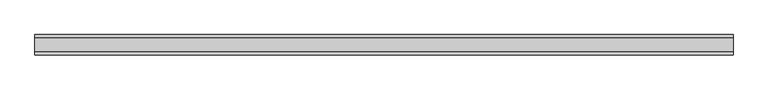
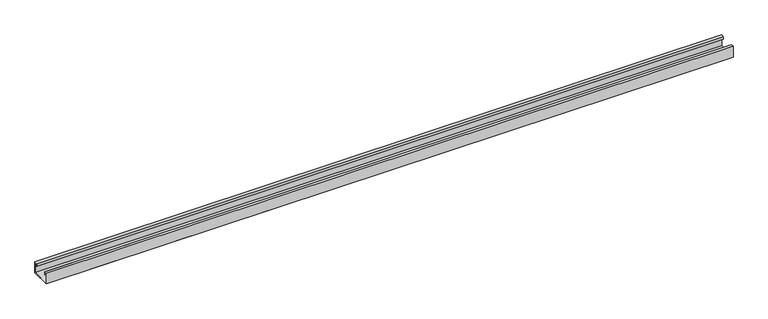
"""IFC4 building model written with IfcOpenShell, lengths in millimetres: proxy geometry, Generic Models 7:Generic Models 1:1:Generic Models 1:1 : Generic Models 7:Generic Models 1:337419:57 : Generic Models 7:Generic Models 1:1:Generic Models 1:1 : Generic Models 7:Generic Models 1:337419:306201."""

from ifc_helpers import new_model, si_unit, frame, origin, place, context, project, spatial, polyline, outline, extrude, source, transform, mapped, element, save


def generic_models_7ddd9d2e(model_context):
    return source(origin(), model_context, "Body", "SweptSolid", [
        extrude(outline(polyline([(-578792.9131695, 2440.1859375), (-579005.2695987, 2440.1859375), (-579005.2695987, 2561.318129), (-578973.5195987, 2561.318129), (-578973.5195987, 2529.568129), (-578976.4229092, 2529.568129), (-578976.4229092, 2558.4148184), (-579002.3662881, 2558.4148184), (-579002.3662881, 2443.0892481), (-578795.8164801, 2443.0892481), (-578795.8164801, 2558.4148184), (-578821.7598589, 2558.4148184), (-578821.7598589, 2529.568129), (-578824.6631695, 2529.568129), (-578824.6631695, 2561.318129), (-578792.9131695, 2561.318129), (-578792.9131695, 2440.1859375)])), frame((588867.6367239, 0.0, 0.0), z_axis=(1.0, 0.0, 0.0), x_axis=(0.0, 1.0, 0.0)), (0.0, 0.0, 1.0), 7315.2),
    ])


if __name__ == "__main__":
    model = new_model("IFC4")
    model_context = context("Model", 3, world=origin())
    ifc_project = project(units=[si_unit("LENGTHUNIT", "METRE", prefix="MILLI")], contexts=[model_context])
    site = spatial("IfcSite", under=ifc_project)
    building = spatial("IfcBuilding", under=site)
    placement = place(None, origin())
    generic_models_shape = generic_models_7ddd9d2e(model_context)
    element("IfcBuildingElementProxy", 1, Name="Generic Models 7:Generic Models 1:1:Generic Models 1:1 : Generic Models 7:Generic Models 1:337419:57 : Generic Models 7:Generic Models 1:1:Generic Models 1:1 : Generic Models 7:Generic Models 1:337419:306201", ObjectType="Generic Models 7:Generic Models 1:1:Generic Models 1:1 : Generic Models 7:Generic Models 1:337419:57 : Generic Models 7:Generic Models 1:1:Generic Models 1:1 : Generic Models 7:Generic Models 1:337419:306201", at=placement, inside=building, context=model_context, shape_type="MappedRepresentation", body=[
        mapped(generic_models_shape, transform((0.0, 0.0, 0.0), x_axis=(1.0, 0.0, 0.0), y_axis=(0.0, 1.0, 0.0), z_axis=(0.0, 0.0, 1.0))),
    ])
    save(model, "model.ifc")

# Revit data of these elements
# Type "Generic Models 7:Generic Models 1:1:Generic Models 1:1 : Generic Models 7:Generic Models 1:337419:57 : Generic Models 7:Generic Models 1:1:Generic Models 1:1 : Generic Models 7:Generic Models 1:337419:306201"
#   NameOverride = "Generic Models 7:Generic Models 1:1:Generic Models 1:1 : Generic Models 7:Generic Models 1:337419:306201"
#   ObjectTypeOverride = "Generic Models 1:1 : Generic Models 7:Generic Models 1:337419"
#   Reference = "Generic Models 1"
#   Tag = "306201"
# Element 1 (IfcBuildingElementProxy, "Generic Models 7:Generic Models 1:1:Generic Models 1:1 : Generic Models 7:Generic Models 1:337419:57 : Generic Models 7:Generic Models 1:1:Generic Models 1:1 : Generic Models 7:Generic Models 1:337419:306201")
#   Materials on its faces: "WRAP CEE GIRT WITH STAINLESS STAIN BRAKE METAL (IF ALUM GASKET AWAY FROM STEEL)"
# Materials
#   "WRAP CEE GIRT WITH STAINLESS STAIN BRAKE METAL (IF ALUM GASKET AWAY FROM STEEL)": class "Unassigned", colour RGB 202 201 200, transparency 0, Cost = 0
